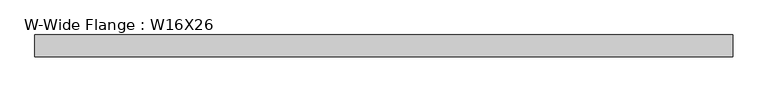
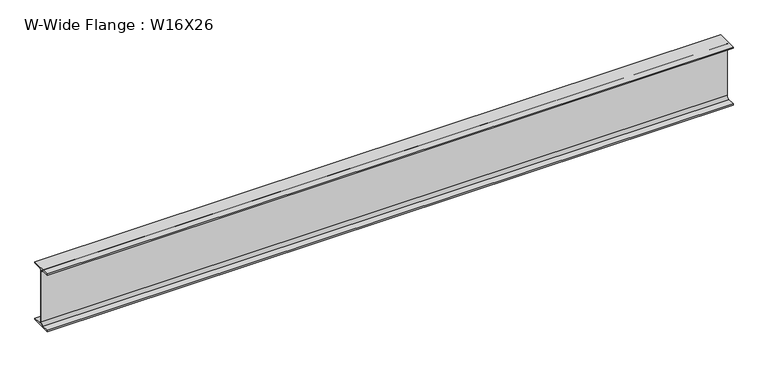
"""IFC4 building model written with IfcOpenShell, lengths in millimetres: beam geometry, W-Wide Flange : W16X26."""

from ifc_helpers import new_model, si_unit, point, frame, frame_2d, origin, place, context, project, spatial, polyline, circle_curve, trimmed, segment, composite_curve, outline, extrude, source, transform, mapped, element, save


def w_wide_flange_w16x26_9b29557f(model_context):
    return source(origin(), model_context, "Body", "SweptSolid", [
        extrude(outline(composite_curve([segment(polyline([(69.85, -190.627), (69.85, -199.39), (-69.85, -199.39), (-69.85, -190.627), (-21.3995, -190.627)]), True, "CONTINUOUS"), segment(trimmed(circle_curve(frame_2d((-21.3995, -172.4025)), 18.2245), [point((-21.3995, -190.627))], [point((-3.175, -172.4025))], True, "CARTESIAN"), True, "CONTINUOUS"), segment(polyline([(-3.175, -172.4025), (-3.175, 172.4025)]), True, "CONTINUOUS"), segment(trimmed(circle_curve(frame_2d((-21.3995, 172.4025)), 18.2245), [point((-3.175, 172.4025))], [point((-21.3995, 190.627))], True, "CARTESIAN"), True, "CONTINUOUS"), segment(polyline([(-21.3995, 190.627), (-69.85, 190.627), (-69.85, 199.39), (69.85, 199.39), (69.85, 190.627), (21.3995, 190.627)]), True, "CONTINUOUS"), segment(trimmed(circle_curve(frame_2d((21.3995, 172.4025)), 18.2245), [point((21.3995, 190.627))], [point((3.175, 172.4025))], True, "CARTESIAN"), True, "CONTINUOUS"), segment(polyline([(3.175, 172.4025), (3.175, -172.4025)]), True, "CONTINUOUS"), segment(trimmed(circle_curve(frame_2d((21.3995, -172.4025)), 18.2245), [point((3.175, -172.4025))], [point((21.3995, -190.627))], True, "CARTESIAN"), True, "CONTINUOUS"), segment(polyline([(21.3995, -190.627), (69.85, -190.627)]), True, "CONTINUOUS")], self_intersect=False)), frame((-2235.2, 0.0, 0.0), z_axis=(1.0, 0.0, 0.0), x_axis=(0.0, 1.0, 0.0)), (0.0, 0.0, 1.0), 4470.4),
    ])


if __name__ == "__main__":
    model = new_model("IFC4")
    model_context = context("Model", 3, world=origin())
    ifc_project = project(units=[si_unit("LENGTHUNIT", "METRE", prefix="MILLI")], contexts=[model_context])
    site = spatial("IfcSite", under=ifc_project)
    building = spatial("IfcBuilding", under=site)
    placement = place(None, origin())
    w_wide_flange_w16x26_shape = w_wide_flange_w16x26_9b29557f(model_context)
    element("IfcBeam", 1, ObjectType="W-Wide Flange : W16X26", at=placement, inside=building, context=model_context, shape_type="MappedRepresentation", body=[
        mapped(w_wide_flange_w16x26_shape, transform((0.0, 0.0, 0.0), x_axis=(1.0, 0.0, 0.0), y_axis=(0.0, 1.0, 0.0), z_axis=(0.0, 0.0, 1.0))),
    ])
    save(model, "model.ifc")

# Revit data of these elements
# Type "W-Wide Flange : W16X26"
#   Assembly Code = "B10"
#   W = 26
#   Length [instance default] = 5' - 0"
#   bf = 0' - 5 1/2"
#   d = 1' - 3.7"
#   k = 0' - 1 1/16"
#   k2 = 0' - 0.7175"
#   tf = 0' - 0.345"
#   tw = 0' - 0 1/4"
#   A = 0.0533333 SF
#   Structural Material [instance default] = Steel ASTM A992
# Element 1 (IfcBeam, "W-Wide Flange : W16X26")
#   Materials on its faces: "Steel ASTM A992"
# Materials
#   "Steel ASTM A992": class "Metal", colour RGB 199 199 199, transparency 0, Description = "Structural steel 50ksi", Cost = 0
